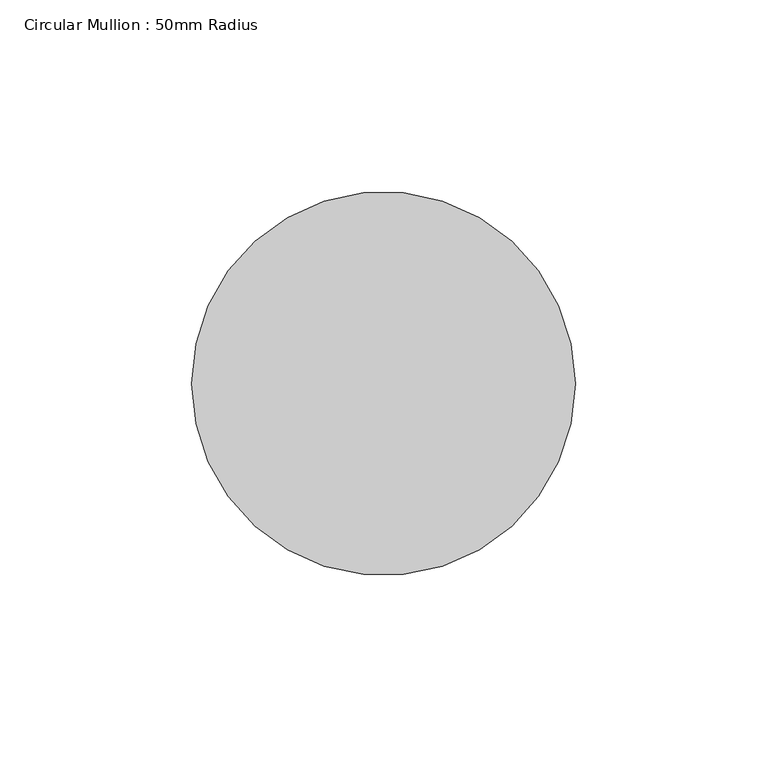
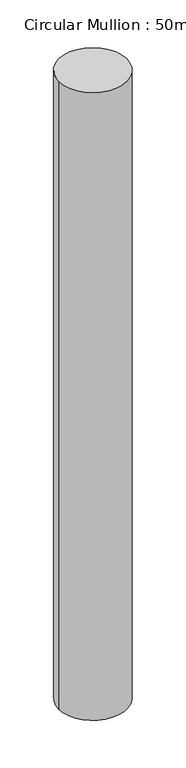
"""IFC4 building model written with IfcOpenShell, lengths in millimetres: member geometry, Circular Mullion : 50mm Radius."""

from ifc_helpers import new_model, si_unit, point, frame, origin, origin_2d, place, context, project, spatial, circle_curve, trimmed, segment, composite_curve, outline, extrude, source, transform, mapped, element, save


def circular_mullion_50mm_radius_c347b794(model_context):
    return source(origin(), model_context, "Body", "SweptSolid", [
        extrude(outline(composite_curve([segment(trimmed(circle_curve(origin_2d(), 50.0), [point((50.0, 0.0))], [point((-50.0, 0.0))], False, "CARTESIAN"), True, "CONTINUOUS"), segment(trimmed(circle_curve(origin_2d(), 50.0), [point((-50.0, 0.0))], [point((50.0, 0.0))], False, "CARTESIAN"), True, "CONTINUOUS")], self_intersect=False)), frame((0.0, 0.0, -974.474483), z_axis=(0.0, 0.0, 1.0), x_axis=(1.0, 0.0, 0.0)), (0.0, 0.0, 1.0), 974.474483),
    ])


if __name__ == "__main__":
    model = new_model("IFC4")
    model_context = context("Model", 3, world=origin())
    ifc_project = project(units=[si_unit("LENGTHUNIT", "METRE", prefix="MILLI")], contexts=[model_context])
    site = spatial("IfcSite", under=ifc_project)
    building = spatial("IfcBuilding", under=site)
    placement = place(None, origin())
    circular_mullion_50mm_radius_shape = circular_mullion_50mm_radius_c347b794(model_context)
    element("IfcMember", 1, ObjectType="Circular Mullion : 50mm Radius", at=placement, inside=building, context=model_context, shape_type="MappedRepresentation", body=[
        mapped(circular_mullion_50mm_radius_shape, transform((0.0, 0.0, 0.0), x_axis=(1.0, 0.0, 0.0), y_axis=(0.0, 1.0, 0.0), z_axis=(0.0, 0.0, 1.0))),
    ])
    save(model, "model.ifc")

# Revit data of these elements
# Type "Circular Mullion : 50mm Radius"
#   built-in parameter 1007350 = 0.164042 (stored number, unit not read)
# Element 1 (IfcMember, "Circular Mullion : 50mm Radius")
#   Materials on its faces: "Aluminium"
# Materials
#   "Aluminium": class "Metal", colour RGB 247 247 247, transparency 0, Description = "Aluminium 6061", Cost = 0
